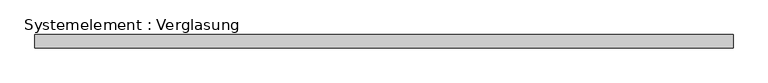
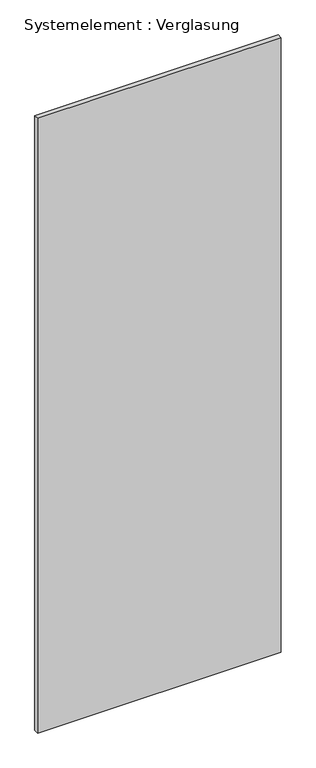
"""IFC4 building model written with IfcOpenShell, lengths in millimetres: plate geometry, Systemelement : Verglasung."""

from ifc_helpers import new_model, si_unit, origin, origin_with_axes, place, context, project, spatial, polyline, outline, extrude, source, transform, mapped, element, save


def systemelement_verglasung_bb89f317(model_context):
    return source(origin(), model_context, "Body", "SweptSolid", [
        extrude(outline(polyline([(794.9747918, -15.0), (-794.9747918, -15.0), (-794.9747918, 15.0), (794.9747918, 15.0), (794.9747918, -15.0)])), origin_with_axes(), (0.0, 0.0, 1.0), 4236.6788019),
    ])


if __name__ == "__main__":
    model = new_model("IFC4")
    model_context = context("Model", 3, world=origin())
    ifc_project = project(units=[si_unit("LENGTHUNIT", "METRE", prefix="MILLI")], contexts=[model_context])
    site = spatial("IfcSite", under=ifc_project)
    building = spatial("IfcBuilding", under=site)
    placement = place(None, origin())
    systemelement_verglasung_shape = systemelement_verglasung_bb89f317(model_context)
    element("IfcPlate", 1, ObjectType="Systemelement : Verglasung", at=placement, inside=building, context=model_context, shape_type="MappedRepresentation", body=[
        mapped(systemelement_verglasung_shape, transform((0.0, 0.0, 0.0), x_axis=(1.0, 0.0, 0.0), y_axis=(0.0, 1.0, 0.0), z_axis=(0.0, 0.0, 1.0))),
    ])
    save(model, "model.ifc")

# Revit data of these elements
# Type "Systemelement : Verglasung"
#   Construction Type Id = "GSP4R"
#   Analytic Construction = "1/8 Zoll Pilkington-Verglasung einfach"
#   Visual Light Transmittance = 0.9
#   Solar Heat Gain Coefficient = 0.86
#   Heat Transfer Coefficient (U) = 6.7069 W/(m²·K)
# Element 1 (IfcPlate, "Systemelement : Verglasung")
#   Materials on its faces: "Glas"
# Materials
#   "Glas": class "Glas", colour RGB 0 0 255, transparency 0.75, Comments = "Render-Darstellung nicht aktualisiert ", Cost = 0
